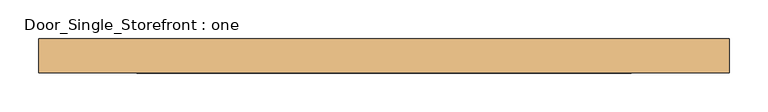
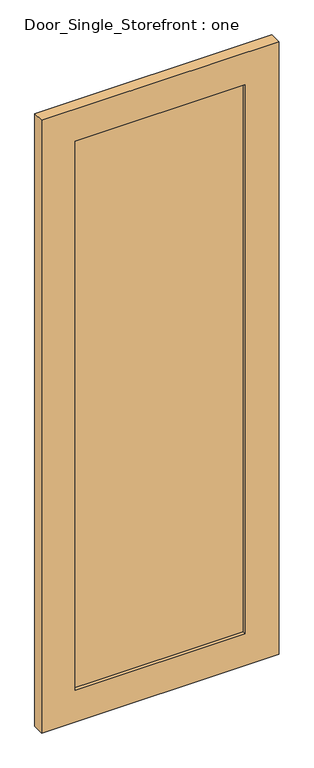
"""IFC4 building model written with IfcOpenShell, lengths in millimetres: door geometry, Door_Single_Storefront : one."""

from ifc_helpers import new_model, si_unit, frame, origin, place, context, project, spatial, polyline, outline, extrude, source, transform, mapped, element, save


def door_single_storefront_one_6aadf17f(model_context):
    return source(origin(), model_context, "Body", "SweptSolid", [
        extrude(outline(polyline([(319.88125, 6.35), (319.88125, -12.7), (-319.88125, -12.7), (-319.88125, 6.35), (319.88125, 6.35)])), frame((0.0, 0.0, 127.0), z_axis=(0.0, 0.0, 1.0), x_axis=(1.0, 0.0, 0.0)), (0.0, 0.0, 1.0), 2184.4),
        extrude(outline(polyline([(2438.4, -446.88125), (0.0, -446.88125), (0.0, 446.88125), (2438.4, 446.88125), (2438.4, -446.88125)]), holes=[polyline([(127.0, 319.88125), (127.0, -319.88125), (2311.4, -319.88125), (2311.4, 319.88125), (127.0, 319.88125)])]), frame((0.0, -25.4, 0.0), z_axis=(0.0, 1.0, 0.0), x_axis=(0.0, 0.0, 1.0)), (0.0, 0.0, 1.0), 44.45),
    ])


if __name__ == "__main__":
    model = new_model("IFC4")
    model_context = context("Model", 3, world=origin())
    ifc_project = project(units=[si_unit("LENGTHUNIT", "METRE", prefix="MILLI")], contexts=[model_context])
    site = spatial("IfcSite", under=ifc_project)
    building = spatial("IfcBuilding", under=site)
    placement = place(None, origin())
    door_single_storefront_one_shape = door_single_storefront_one_6aadf17f(model_context)
    element("IfcDoor", 1, ObjectType="Door_Single_Storefront : one", at=placement, inside=building, context=model_context, shape_type="MappedRepresentation", body=[
        mapped(door_single_storefront_one_shape, transform((0.0, 0.0, 0.0), x_axis=(1.0, 0.0, 0.0), y_axis=(0.0, 1.0, 0.0), z_axis=(0.0, 0.0, 1.0))),
    ])
    save(model, "model.ifc")

# Revit data of these elements
# Type "Door_Single_Storefront : one"
#   Type Mark = "27"
#   Analytic Construction = "<None>"
#   Stile_Width = 0' - 5"
#   Door_Thickness = 0' - 1 3/4"
#   Door_Offset = 0' - 1"
#   Glass_Material = SAFETY GLAZING
#   Frame_Material = INTERIOR GRADE ALUMINUM STOREFRONT W/ SAFETY GLAZING
#   Function = (empty or 0)
# Element 1 (IfcDoor, "Door_Single_Storefront : one")
#   Materials on its faces: "INTERIOR GRADE ALUMINUM STOREFRONT W/ SAFETY GLAZING", "SAFETY GLAZING"
# Materials
#   "SAFETY GLAZING": class "Glass", colour RGB 142 168 196, transparency 0.75, Description = "Soda Lime Glass", Cost = 0
#   "INTERIOR GRADE ALUMINUM STOREFRONT W/ SAFETY GLAZING": class "Metal", colour RGB 226 226 226, transparency 0, Description = "Aluminum 6061", Cost = 0
